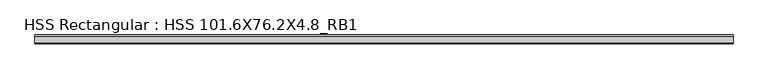
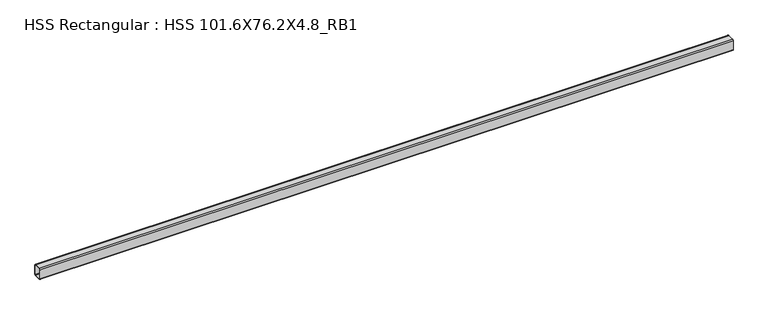
"""IFC4 building model written with IfcOpenShell, lengths in millimetres: beam geometry, HSS Rectangular : HSS 101.6X76.2X4.8_RB1."""

import ifcopenshell
import ifcopenshell.guid

model = None  # the IFC model being written
_history = None  # IfcOwnerHistory: only IFC2X3 demands one
_inside = {}  # id of a spatial element -> (the spatial element, [elements in it])
_under = {}  # id of a project, library or spatial element -> (it, [spatial elements below it])
_declared = {}  # id of a project -> (the project, [libraries it declares])
_typed = {}  # id of a type object -> (the type object, [elements of that type])
_made_of = {}  # id of a material, layer set ... -> (it, [elements and type objects made of it])


def new_model(schema):
    """Start an empty IFC model of exactly this schema.

    Asked for "IFC4X3", IfcOpenShell would pick the latest addendum, in which some entities
    have other attributes; the version numbers below select the first issue.
    IFC2X3 requires an IfcOwnerHistory on every rooted entity: one is made here for all.
    """
    global model, _history
    if schema == "IFC4X3":
        model = ifcopenshell.file(schema_version=(4, 3, 0, 0))
    else:
        model = ifcopenshell.file(schema=schema)
    _inside.clear()
    _under.clear()
    _declared.clear()
    _typed.clear()
    _made_of.clear()
    _history = None
    if model.schema == "IFC2X3":
        org = make("IfcOrganization", Name="unknown")
        user = make(
            "IfcPersonAndOrganization",
            ThePerson=make("IfcPerson", FamilyName="unknown"),
            TheOrganization=org,
        )
        app = make(
            "IfcApplication",
            ApplicationDeveloper=org,
            Version="unknown",
            ApplicationFullName="unknown",
            ApplicationIdentifier="unknown",
        )
        _history = make(
            "IfcOwnerHistory",
            OwningUser=user,
            OwningApplication=app,
            ChangeAction="ADDED",
            CreationDate=0,
        )
    return model


def make(cls, **values):
    """One entity of the class cls with the attributes given. An attribute that is None is left unset."""
    return model.create_entity(
        cls, **{name: value for name, value in values.items() if value is not None}
    )


def rooted(cls, **values):
    """An entity with a GlobalId (a new one), such as an element, a storey or a relation."""
    return make(cls, GlobalId=ifcopenshell.guid.new(), OwnerHistory=_history, **values)


def si_unit(unit_type, name, prefix=None):
    """IfcSIUnit, for example si_unit("LENGTHUNIT", "METRE", prefix="MILLI")."""
    return make("IfcSIUnit", UnitType=unit_type, Prefix=prefix, Name=name)


def assignment(units):
    """IfcUnitAssignment: the units of a project."""
    return None if units is None else make("IfcUnitAssignment", Units=units)


def point(xyz):
    """IfcCartesianPoint."""
    return None if xyz is None else make("IfcCartesianPoint", Coordinates=xyz)


def direction(xyz):
    """IfcDirection."""
    return None if xyz is None else make("IfcDirection", DirectionRatios=xyz)


def frame(location, z_axis=None, x_axis=None):
    """IfcAxis2Placement3D, a coordinate frame: its origin and axes. An axis left out is left unset."""
    return make(
        "IfcAxis2Placement3D",
        Location=point(location),
        Axis=direction(z_axis),
        RefDirection=direction(x_axis),
    )


def frame_2d(location, x_axis=None):
    """IfcAxis2Placement2D, a coordinate frame in the plane: its origin and x axis."""
    return make(
        "IfcAxis2Placement2D", Location=point(location), RefDirection=direction(x_axis)
    )


def origin():
    """The frame at (0, 0, 0) with its axes left unset."""
    return frame((0.0, 0.0, 0.0))


def place(relative_to, where):
    """IfcLocalPlacement: puts the frame where relative to a parent placement (None: the world)."""
    return make(
        "IfcLocalPlacement", PlacementRelTo=relative_to, RelativePlacement=where
    )


def context(
    kind, dimensions, precision=None, world=None, true_north=None, identifier=None
):
    """IfcGeometricRepresentationContext, for example the 3D "Model" context."""
    return make(
        "IfcGeometricRepresentationContext",
        ContextIdentifier=identifier,
        ContextType=kind,
        CoordinateSpaceDimension=dimensions,
        Precision=precision,
        WorldCoordinateSystem=world,
        TrueNorth=true_north,
    )


def project(units=None, contexts=None):
    """IfcProject with its units and contexts."""
    return rooted(
        "IfcProject",
        Name="project",
        RepresentationContexts=contexts,
        UnitsInContext=assignment(units),
    )


def spatial(cls, under=None, at=None, **own):
    """A site, building, storey or space (cls), placed at a placement, below another one or the project."""
    s = rooted(cls, ObjectPlacement=at, **own)
    if under is not None:
        _under.setdefault(under.id(), (under, []))[1].append(s)
    return s


def polyline(points):
    """IfcPolyline through the points."""
    return make("IfcPolyline", Points=[point(p) for p in points])


def circle_curve(where, radius):
    """IfcCircle in the frame where."""
    return make("IfcCircle", Position=where, Radius=radius)


def trimmed(basis, trim1, trim2, sense, master):
    """IfcTrimmedCurve: the piece of a basis curve between two trims."""
    return make(
        "IfcTrimmedCurve",
        BasisCurve=basis,
        Trim1=trim1,
        Trim2=trim2,
        SenseAgreement=sense,
        MasterRepresentation=master,
    )


def segment(curve, same_sense, transition):
    """IfcCompositeCurveSegment."""
    return make(
        "IfcCompositeCurveSegment",
        Transition=transition,
        SameSense=same_sense,
        ParentCurve=curve,
    )


def composite_curve(segments, self_intersect=None):
    """IfcCompositeCurve: segments joined end to end."""
    return make("IfcCompositeCurve", Segments=segments, SelfIntersect=self_intersect)


def outline(outer, holes=None, kind="AREA"):
    """IfcArbitraryClosedProfileDef: a profile drawn as a closed curve; with holes, ...WithVoids."""
    if holes is None:
        return make("IfcArbitraryClosedProfileDef", ProfileType=kind, OuterCurve=outer)
    return make(
        "IfcArbitraryProfileDefWithVoids",
        ProfileType=kind,
        OuterCurve=outer,
        InnerCurves=holes,
    )


def extrude(swept, where, along, depth):
    """IfcExtrudedAreaSolid: the profile swept, set in the frame where, extruded along a direction by depth."""
    return make(
        "IfcExtrudedAreaSolid",
        SweptArea=swept,
        Position=where,
        ExtrudedDirection=direction(along),
        Depth=depth,
    )


def shape(context_of_items, identifier, shape_type, items):
    """IfcShapeRepresentation: the items that make up one representation, for example the "Body"."""
    return make(
        "IfcShapeRepresentation",
        ContextOfItems=context_of_items,
        RepresentationIdentifier=identifier,
        RepresentationType=shape_type,
        Items=items,
    )


def source(mapping_origin, context_of_items, identifier, shape_type, items):
    """IfcRepresentationMap: a shape defined once, which mapped items show again and again."""
    return make(
        "IfcRepresentationMap",
        MappingOrigin=mapping_origin,
        MappedRepresentation=shape(context_of_items, identifier, shape_type, items),
    )


def transform(
    local_origin,
    x_axis=None,
    y_axis=None,
    z_axis=None,
    scale=None,
    scale2=None,
    scale3=None,
    uniform=True,
):
    """IfcCartesianTransformationOperator3D, or its non-uniform kind. x_axis, y_axis, z_axis: its Axis1, 2, 3."""
    if uniform:
        return make(
            "IfcCartesianTransformationOperator3D",
            Axis1=direction(x_axis),
            Axis2=direction(y_axis),
            LocalOrigin=point(local_origin),
            Scale=scale,
            Axis3=direction(z_axis),
        )
    return make(
        "IfcCartesianTransformationOperator3DnonUniform",
        Axis1=direction(x_axis),
        Axis2=direction(y_axis),
        LocalOrigin=point(local_origin),
        Scale=scale,
        Axis3=direction(z_axis),
        Scale2=scale2,
        Scale3=scale3,
    )


def mapped(mapping_source, mapping_target):
    """IfcMappedItem: shows the shape of a source again, moved by a transform."""
    return make(
        "IfcMappedItem", MappingSource=mapping_source, MappingTarget=mapping_target
    )


def made_of(thing, what):
    """Note that an element or type object is made of a material, layer set ...; save() writes the relation."""
    if what is not None:
        _made_of.setdefault(what.id(), (what, []))[1].append(thing)
    return thing


def element(
    cls,
    number,
    at=None,
    inside=None,
    cuts=None,
    type_object=None,
    material=None,
    context=None,
    identifier="Body",
    shape_type=None,
    held_by="IfcProductDefinitionShape",
    body=None,
    shapes=None,
    **own,
):
    """One element of the class cls, such as IfcWall. Its Tag is "e" and its number.

    at: its placement. inside: the storey or other place that contains it. cuts: it is an
    opening in that element (IfcRelVoidsElement). A single representation is given by context,
    identifier, shape_type and body (its items); several are given by shapes. held_by: the class
    of the entity that holds the representations. save() writes the other relations.
    """
    e = rooted(cls, Tag="e%d" % number, ObjectPlacement=at, **own)
    if body is not None:
        shapes = [shape(context, identifier, shape_type, body)]
    if shapes is not None:
        e.Representation = make(held_by, Representations=shapes)
    if inside is not None:
        _inside.setdefault(inside.id(), (inside, []))[1].append(e)
    if cuts is not None:
        rooted(
            "IfcRelVoidsElement", RelatingBuildingElement=cuts, RelatedOpeningElement=e
        )
    if type_object is not None:
        _typed.setdefault(type_object.id(), (type_object, []))[1].append(e)
    return made_of(e, material)


def aggregate(whole, parts):
    """IfcRelAggregates: a whole, such as a stair, and the parts it consists of."""
    return rooted("IfcRelAggregates", RelatingObject=whole, RelatedObjects=parts)


def save(model, path):
    """Write the relations noted so far, then the file.

    IfcRelAggregates (storeys below a building ...), IfcRelContainedInSpatialStructure (elements
    in a storey), IfcRelDefinesByType, IfcRelAssociatesMaterial and IfcRelDeclares: one each for
    every whole, place, type object, material and project.
    """
    for whole, parts in _under.values():
        aggregate(whole, parts)
    for where, things in _inside.values():
        rooted(
            "IfcRelContainedInSpatialStructure",
            RelatedElements=things,
            RelatingStructure=where,
        )
    for kind, things in _typed.values():
        rooted("IfcRelDefinesByType", RelatedObjects=things, RelatingType=kind)
    for what, things in _made_of.values():
        rooted("IfcRelAssociatesMaterial", RelatedObjects=things, RelatingMaterial=what)
    for by, libraries in _declared.values():
        rooted("IfcRelDeclares", RelatingContext=by, RelatedDefinitions=libraries)
    model.write(path)


def hss_rectangular_hss_101_6x76_2x4_8_rb1_0317c0dd(model_context):
    return source(origin(), model_context, "Body", "SweptSolid", [
        extrude(outline(composite_curve([segment(polyline([(38.1, 41.275), (38.1, -41.275)]), True, "CONTINUOUS"), segment(trimmed(circle_curve(frame_2d((28.575, -41.275)), 9.525), [point((38.1, -41.275))], [point((28.575, -50.8))], False, "CARTESIAN"), True, "CONTINUOUS"), segment(polyline([(28.575, -50.8), (-28.575, -50.8)]), True, "CONTINUOUS"), segment(trimmed(circle_curve(frame_2d((-28.575, -41.275)), 9.525), [point((-28.575, -50.8))], [point((-38.1, -41.275))], False, "CARTESIAN"), True, "CONTINUOUS"), segment(polyline([(-38.1, -41.275), (-38.1, 41.275)]), True, "CONTINUOUS"), segment(trimmed(circle_curve(frame_2d((-28.575, 41.275)), 9.525), [point((-38.1, 41.275))], [point((-28.575, 50.8))], False, "CARTESIAN"), True, "CONTINUOUS"), segment(polyline([(-28.575, 50.8), (28.575, 50.8)]), True, "CONTINUOUS"), segment(trimmed(circle_curve(frame_2d((28.575, 41.275)), 9.525), [point((28.575, 50.8))], [point((38.1, 41.275))], False, "CARTESIAN"), True, "CONTINUOUS")], self_intersect=False), holes=[composite_curve([segment(trimmed(circle_curve(frame_2d((-28.575, 41.275)), 4.7625), [point((-28.575, 46.0375))], [point((-33.3375, 41.275))], True, "CARTESIAN"), True, "CONTINUOUS"), segment(polyline([(-33.3375, 41.275), (-33.3375, -41.275)]), True, "CONTINUOUS"), segment(trimmed(circle_curve(frame_2d((-28.575, -41.275)), 4.7625), [point((-33.3375, -41.275))], [point((-28.575, -46.0375))], True, "CARTESIAN"), True, "CONTINUOUS"), segment(polyline([(-28.575, -46.0375), (28.575, -46.0375)]), True, "CONTINUOUS"), segment(trimmed(circle_curve(frame_2d((28.575, -41.275)), 4.7625), [point((28.575, -46.0375))], [point((33.3375, -41.275))], True, "CARTESIAN"), True, "CONTINUOUS"), segment(polyline([(33.3375, -41.275), (33.3375, 41.275)]), True, "CONTINUOUS"), segment(trimmed(circle_curve(frame_2d((28.575, 41.275)), 4.7625), [point((33.3375, 41.275))], [point((28.575, 46.0375))], True, "CARTESIAN"), True, "CONTINUOUS"), segment(polyline([(28.575, 46.0375), (-28.575, 46.0375)]), True, "CONTINUOUS")], self_intersect=False)]), frame((-7500.0, 0.0, 0.0), z_axis=(1.0, 0.0, 0.0), x_axis=(0.0, 1.0, 0.0)), (0.0, 0.0, 1.0), 6077.1944025),
    ])


if __name__ == "__main__":
    model = new_model("IFC4")
    model_context = context("Model", 3, world=origin())
    ifc_project = project(units=[si_unit("LENGTHUNIT", "METRE", prefix="MILLI")], contexts=[model_context])
    site = spatial("IfcSite", under=ifc_project)
    building = spatial("IfcBuilding", under=site)
    placement = place(None, origin())
    hss_rectangular_hss_101_6x76_2x4_8_rb1_shape = hss_rectangular_hss_101_6x76_2x4_8_rb1_0317c0dd(model_context)
    element("IfcBeam", 1, ObjectType="HSS Rectangular : HSS 101.6X76.2X4.8_RB1", at=placement, inside=building, context=model_context, shape_type="MappedRepresentation", body=[
        mapped(hss_rectangular_hss_101_6x76_2x4_8_rb1_shape, transform((0.0, 0.0, 0.0), x_axis=(1.0, 0.0, 0.0), y_axis=(0.0, 1.0, 0.0), z_axis=(0.0, 0.0, 1.0))),
    ])
    save(model, "model.ifc")

# Revit data of these elements
# Type "HSS Rectangular : HSS 101.6X76.2X4.8_RB1"
#   Section Name Key = "HSS 4X3X3/16"
#   Assembly Code = "B10"
#   Width = 7.62 cm
#   Wall Nominal Thickness = 0.4763 cm
#   Wall Design Thickness = 0.442 cm
#   Torsional Moment of Inertia = 260.561 cm⁴
#   Torsional Modulus = 61.2876 cm³
#   Section Area = 14.4516 cm²
#   Plastic Modulus weak axis = 40.3122 cm³
#   Plastic Modulus strong axis = 49.1612 cm³
#   Perimeter = 0.881482 m²/m
#   Outer Fillet = 0.9525 cm
#   Nominal Weight = 12.1285 kgf/m
#   Moment of Inertia weak axis = 131.529 cm⁴
#   Moment of Inertia strong axis = 205.202 cm⁴
#   Inner Fillet = 0.4763 cm
#   Height = 10.16 cm
#   Elastic Modulus weak axis = 34.4128 cm³
#   Elastic Modulus strong axis = 40.476 cm³
#   Centroid Vertical = 5.08 cm
#   Centroid Horizontal = 3.81 cm
#   Length [instance default] = 1524 mm
#   Structural Material [instance default] = Steel ASTM A500, Grade B, Rectangular and Square
#   Principal Axes Angle = 0
# Element 1 (IfcBeam, "HSS Rectangular : HSS 101.6X76.2X4.8_RB1")
#   Structural Material = Steel ASTM A992
#   Materials on its faces: "Steel ASTM A992"
# Materials
#   "Steel ASTM A500, Grade B, Rectangular and Square": class "Metal", colour RGB 199 199 199, transparency 0, Description = "Carbon steel", Cost = 0
#   "Steel ASTM A992": class "Metal", colour RGB 199 199 199, transparency 0, Description = "Structural steel 50ksi", Cost = 0
